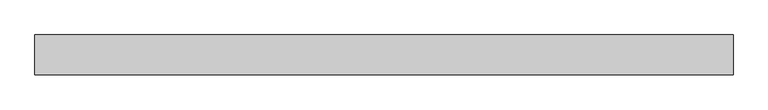
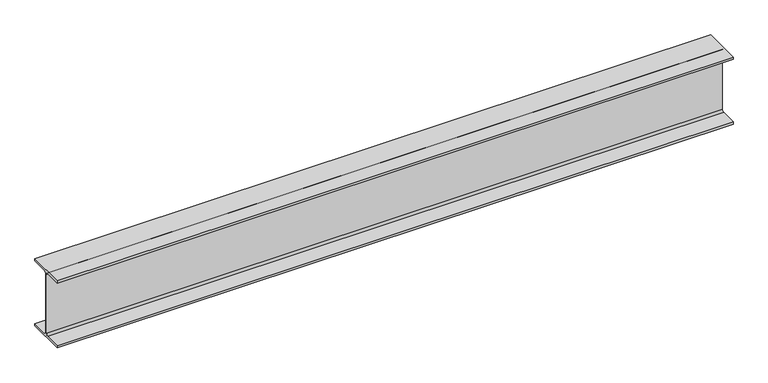
"""IFC4 building model written with IfcOpenShell, lengths in millimetres: beam geometry, Old_Steel Beam_H-KSD3502 : H_SB_ASB_H-250×125x6x9."""

from ifc_helpers import new_model, si_unit, point, frame, frame_2d, origin, place, context, project, spatial, polyline, circle_curve, trimmed, segment, composite_curve, outline, extrude, source, transform, mapped, element, save


def beam_680f737e(model_context):
    return source(origin(), model_context, "Body", "SweptSolid", [
        extrude(outline(composite_curve([segment(polyline([(82.5, -141.5), (82.5, -151.7), (-82.5, -151.7), (-82.5, -141.5), (-11.9, -141.5)]), True, "CONTINUOUS"), segment(trimmed(circle_curve(frame_2d((-11.9, -132.6)), 8.9), [point((-11.9, -141.5))], [point((-3.0, -132.6))], True, "CARTESIAN"), True, "CONTINUOUS"), segment(polyline([(-3.0, -132.6), (-3.0, 132.6)]), True, "CONTINUOUS"), segment(trimmed(circle_curve(frame_2d((-11.9, 132.6)), 8.9), [point((-3.0, 132.6))], [point((-11.9, 141.5))], True, "CARTESIAN"), True, "CONTINUOUS"), segment(polyline([(-11.9, 141.5), (-82.5, 141.5), (-82.5, 151.7), (82.5, 151.7), (82.5, 141.5), (11.9, 141.5)]), True, "CONTINUOUS"), segment(trimmed(circle_curve(frame_2d((11.9, 132.6)), 8.9), [point((11.9, 141.5))], [point((3.0, 132.6))], True, "CARTESIAN"), True, "CONTINUOUS"), segment(polyline([(3.0, 132.6), (3.0, -132.6)]), True, "CONTINUOUS"), segment(trimmed(circle_curve(frame_2d((11.9, -132.6)), 8.9), [point((3.0, -132.6))], [point((11.9, -141.5))], True, "CARTESIAN"), True, "CONTINUOUS"), segment(polyline([(11.9, -141.5), (82.5, -141.5)]), True, "CONTINUOUS")], self_intersect=False)), frame((-1404.8, 0.0, 0.0), z_axis=(1.0, 0.0, 0.0), x_axis=(0.0, 1.0, 0.0)), (0.0, 0.0, 1.0), 2892.0999994),
    ])


if __name__ == "__main__":
    model = new_model("IFC4")
    model_context = context("Model", 3, world=origin())
    ifc_project = project(units=[si_unit("LENGTHUNIT", "METRE", prefix="MILLI")], contexts=[model_context])
    site = spatial("IfcSite", under=ifc_project)
    building = spatial("IfcBuilding", under=site)
    placement = place(None, origin())
    beam_shape = beam_680f737e(model_context)
    element("IfcBeam", 1, ObjectType="Old_Steel Beam_H-KSD3502 : H_SB_ASB_H-250×125x6x9", at=placement, inside=building, context=model_context, shape_type="MappedRepresentation", body=[
        mapped(beam_shape, transform((0.0, 0.0, 0.0), x_axis=(1.0, 0.0, 0.0), y_axis=(0.0, 1.0, 0.0), z_axis=(0.0, 0.0, 1.0))),
    ])
    save(model, "model.ifc")

# Revit data of these elements
# Type "Old_Steel Beam_H-KSD3502 : H_SB_ASB_H-250×125x6x9"
#   Width = 12.5 cm
#   Web Thickness = 0.6 cm
#   Web Fillet = 1.2 cm
#   Warping Constant = 42539.8 cm⁶
#   Torsional Moment of Inertia = 7.8102 cm⁴
#   Torsional Modulus = 1.0 cm³
#   Section Area = 37.66 cm²
#   Plastic Modulus weak axis = 73.1 cm³
#   Plastic Modulus strong axis = 366.0 cm³
#   Perimeter = 0.97 m²/m
#   Nominal Weight = 29.60 kgf/m
#   Moment of Inertia weak axis = 294.00 cm⁴
#   Moment of Inertia strong axis = 4050.00 cm⁴
#   Height = 25.0 cm
#   Flange Thickness = 0.9 cm
#   Elastic Modulus weak axis = 47.0 cm³
#   Elastic Modulus strong axis = 324.0 cm³
#   Centroid Vertical = 12.5 cm
#   Centroid Horizontal = 6.25 cm
#   Length [instance default] = 1.5240 m
#   Structural Material [instance default] = Steel, 45-345
#   Assembly Code = ""
# Element 1 (IfcBeam, "Old_Steel Beam_H-KSD3502 : H_SB_ASB_H-250×125x6x9")
#   Structural Material = none
# Materials
#   "Steel, 45-345": class "Metal", colour RGB 189 187 185, transparency 0, Description = "Steel 345 MPa", Cost = 0
